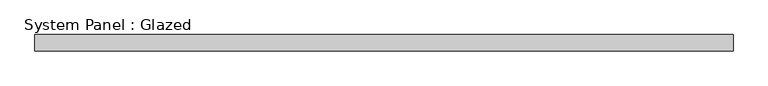
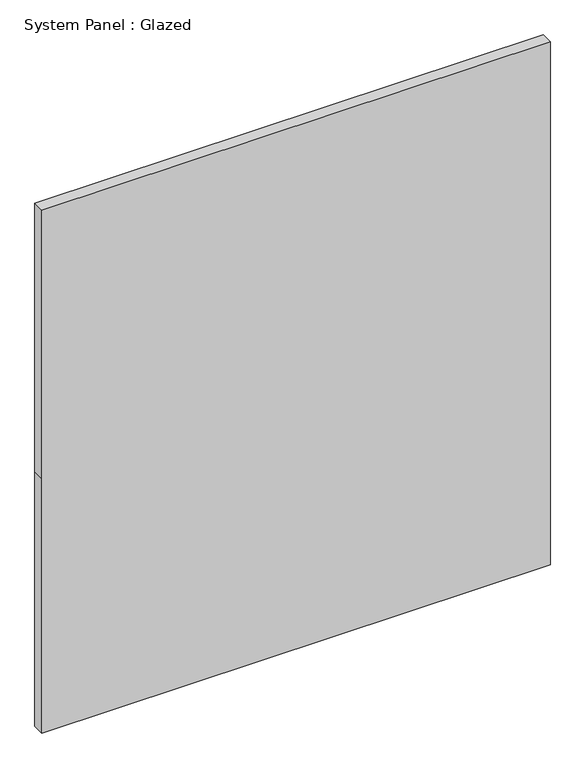
"""IFC4 building model written with IfcOpenShell, lengths in millimetres: plate geometry, System Panel : Glazed."""

import ifcopenshell
import ifcopenshell.guid

model = None  # the IFC model being written
_history = None  # IfcOwnerHistory: only IFC2X3 demands one
_inside = {}  # id of a spatial element -> (the spatial element, [elements in it])
_under = {}  # id of a project, library or spatial element -> (it, [spatial elements below it])
_declared = {}  # id of a project -> (the project, [libraries it declares])
_typed = {}  # id of a type object -> (the type object, [elements of that type])
_made_of = {}  # id of a material, layer set ... -> (it, [elements and type objects made of it])


def new_model(schema):
    """Start an empty IFC model of exactly this schema.

    Asked for "IFC4X3", IfcOpenShell would pick the latest addendum, in which some entities
    have other attributes; the version numbers below select the first issue.
    IFC2X3 requires an IfcOwnerHistory on every rooted entity: one is made here for all.
    """
    global model, _history
    if schema == "IFC4X3":
        model = ifcopenshell.file(schema_version=(4, 3, 0, 0))
    else:
        model = ifcopenshell.file(schema=schema)
    _inside.clear()
    _under.clear()
    _declared.clear()
    _typed.clear()
    _made_of.clear()
    _history = None
    if model.schema == "IFC2X3":
        org = make("IfcOrganization", Name="unknown")
        user = make(
            "IfcPersonAndOrganization",
            ThePerson=make("IfcPerson", FamilyName="unknown"),
            TheOrganization=org,
        )
        app = make(
            "IfcApplication",
            ApplicationDeveloper=org,
            Version="unknown",
            ApplicationFullName="unknown",
            ApplicationIdentifier="unknown",
        )
        _history = make(
            "IfcOwnerHistory",
            OwningUser=user,
            OwningApplication=app,
            ChangeAction="ADDED",
            CreationDate=0,
        )
    return model


def make(cls, **values):
    """One entity of the class cls with the attributes given. An attribute that is None is left unset."""
    return model.create_entity(
        cls, **{name: value for name, value in values.items() if value is not None}
    )


def rooted(cls, **values):
    """An entity with a GlobalId (a new one), such as an element, a storey or a relation."""
    return make(cls, GlobalId=ifcopenshell.guid.new(), OwnerHistory=_history, **values)


def si_unit(unit_type, name, prefix=None):
    """IfcSIUnit, for example si_unit("LENGTHUNIT", "METRE", prefix="MILLI")."""
    return make("IfcSIUnit", UnitType=unit_type, Prefix=prefix, Name=name)


def assignment(units):
    """IfcUnitAssignment: the units of a project."""
    return None if units is None else make("IfcUnitAssignment", Units=units)


def point(xyz):
    """IfcCartesianPoint."""
    return None if xyz is None else make("IfcCartesianPoint", Coordinates=xyz)


def direction(xyz):
    """IfcDirection."""
    return None if xyz is None else make("IfcDirection", DirectionRatios=xyz)


def frame(location, z_axis=None, x_axis=None):
    """IfcAxis2Placement3D, a coordinate frame: its origin and axes. An axis left out is left unset."""
    return make(
        "IfcAxis2Placement3D",
        Location=point(location),
        Axis=direction(z_axis),
        RefDirection=direction(x_axis),
    )


def origin():
    """The frame at (0, 0, 0) with its axes left unset."""
    return frame((0.0, 0.0, 0.0))


def place(relative_to, where):
    """IfcLocalPlacement: puts the frame where relative to a parent placement (None: the world)."""
    return make(
        "IfcLocalPlacement", PlacementRelTo=relative_to, RelativePlacement=where
    )


def context(
    kind, dimensions, precision=None, world=None, true_north=None, identifier=None
):
    """IfcGeometricRepresentationContext, for example the 3D "Model" context."""
    return make(
        "IfcGeometricRepresentationContext",
        ContextIdentifier=identifier,
        ContextType=kind,
        CoordinateSpaceDimension=dimensions,
        Precision=precision,
        WorldCoordinateSystem=world,
        TrueNorth=true_north,
    )


def project(units=None, contexts=None):
    """IfcProject with its units and contexts."""
    return rooted(
        "IfcProject",
        Name="project",
        RepresentationContexts=contexts,
        UnitsInContext=assignment(units),
    )


def spatial(cls, under=None, at=None, **own):
    """A site, building, storey or space (cls), placed at a placement, below another one or the project."""
    s = rooted(cls, ObjectPlacement=at, **own)
    if under is not None:
        _under.setdefault(under.id(), (under, []))[1].append(s)
    return s


def polyline(points):
    """IfcPolyline through the points."""
    return make("IfcPolyline", Points=[point(p) for p in points])


def outline(outer, holes=None, kind="AREA"):
    """IfcArbitraryClosedProfileDef: a profile drawn as a closed curve; with holes, ...WithVoids."""
    if holes is None:
        return make("IfcArbitraryClosedProfileDef", ProfileType=kind, OuterCurve=outer)
    return make(
        "IfcArbitraryProfileDefWithVoids",
        ProfileType=kind,
        OuterCurve=outer,
        InnerCurves=holes,
    )


def extrude(swept, where, along, depth):
    """IfcExtrudedAreaSolid: the profile swept, set in the frame where, extruded along a direction by depth."""
    return make(
        "IfcExtrudedAreaSolid",
        SweptArea=swept,
        Position=where,
        ExtrudedDirection=direction(along),
        Depth=depth,
    )


def shape(context_of_items, identifier, shape_type, items):
    """IfcShapeRepresentation: the items that make up one representation, for example the "Body"."""
    return make(
        "IfcShapeRepresentation",
        ContextOfItems=context_of_items,
        RepresentationIdentifier=identifier,
        RepresentationType=shape_type,
        Items=items,
    )


def source(mapping_origin, context_of_items, identifier, shape_type, items):
    """IfcRepresentationMap: a shape defined once, which mapped items show again and again."""
    return make(
        "IfcRepresentationMap",
        MappingOrigin=mapping_origin,
        MappedRepresentation=shape(context_of_items, identifier, shape_type, items),
    )


def transform(
    local_origin,
    x_axis=None,
    y_axis=None,
    z_axis=None,
    scale=None,
    scale2=None,
    scale3=None,
    uniform=True,
):
    """IfcCartesianTransformationOperator3D, or its non-uniform kind. x_axis, y_axis, z_axis: its Axis1, 2, 3."""
    if uniform:
        return make(
            "IfcCartesianTransformationOperator3D",
            Axis1=direction(x_axis),
            Axis2=direction(y_axis),
            LocalOrigin=point(local_origin),
            Scale=scale,
            Axis3=direction(z_axis),
        )
    return make(
        "IfcCartesianTransformationOperator3DnonUniform",
        Axis1=direction(x_axis),
        Axis2=direction(y_axis),
        LocalOrigin=point(local_origin),
        Scale=scale,
        Axis3=direction(z_axis),
        Scale2=scale2,
        Scale3=scale3,
    )


def mapped(mapping_source, mapping_target):
    """IfcMappedItem: shows the shape of a source again, moved by a transform."""
    return make(
        "IfcMappedItem", MappingSource=mapping_source, MappingTarget=mapping_target
    )


def made_of(thing, what):
    """Note that an element or type object is made of a material, layer set ...; save() writes the relation."""
    if what is not None:
        _made_of.setdefault(what.id(), (what, []))[1].append(thing)
    return thing


def element(
    cls,
    number,
    at=None,
    inside=None,
    cuts=None,
    type_object=None,
    material=None,
    context=None,
    identifier="Body",
    shape_type=None,
    held_by="IfcProductDefinitionShape",
    body=None,
    shapes=None,
    **own,
):
    """One element of the class cls, such as IfcWall. Its Tag is "e" and its number.

    at: its placement. inside: the storey or other place that contains it. cuts: it is an
    opening in that element (IfcRelVoidsElement). A single representation is given by context,
    identifier, shape_type and body (its items); several are given by shapes. held_by: the class
    of the entity that holds the representations. save() writes the other relations.
    """
    e = rooted(cls, Tag="e%d" % number, ObjectPlacement=at, **own)
    if body is not None:
        shapes = [shape(context, identifier, shape_type, body)]
    if shapes is not None:
        e.Representation = make(held_by, Representations=shapes)
    if inside is not None:
        _inside.setdefault(inside.id(), (inside, []))[1].append(e)
    if cuts is not None:
        rooted(
            "IfcRelVoidsElement", RelatingBuildingElement=cuts, RelatedOpeningElement=e
        )
    if type_object is not None:
        _typed.setdefault(type_object.id(), (type_object, []))[1].append(e)
    return made_of(e, material)


def aggregate(whole, parts):
    """IfcRelAggregates: a whole, such as a stair, and the parts it consists of."""
    return rooted("IfcRelAggregates", RelatingObject=whole, RelatedObjects=parts)


def save(model, path):
    """Write the relations noted so far, then the file.

    IfcRelAggregates (storeys below a building ...), IfcRelContainedInSpatialStructure (elements
    in a storey), IfcRelDefinesByType, IfcRelAssociatesMaterial and IfcRelDeclares: one each for
    every whole, place, type object, material and project.
    """
    for whole, parts in _under.values():
        aggregate(whole, parts)
    for where, things in _inside.values():
        rooted(
            "IfcRelContainedInSpatialStructure",
            RelatedElements=things,
            RelatingStructure=where,
        )
    for kind, things in _typed.values():
        rooted("IfcRelDefinesByType", RelatedObjects=things, RelatingType=kind)
    for what, things in _made_of.values():
        rooted("IfcRelAssociatesMaterial", RelatedObjects=things, RelatingMaterial=what)
    for by, libraries in _declared.values():
        rooted("IfcRelDeclares", RelatingContext=by, RelatedDefinitions=libraries)
    model.write(path)


def system_panel_glazed_b3c6389f(model_context):
    return source(origin(), model_context, "Body", "SweptSolid", [
        extrude(outline(polyline([(0.0, -546.4175), (0.0, 546.4175), (577.85, 546.4175), (1187.45, 546.4175), (1187.45, -546.4175), (577.85, -546.4175), (0.0, -546.4175)])), frame((0.0, -44.45, 0.0), z_axis=(0.0, 1.0, 0.0), x_axis=(0.0, 0.0, 1.0)), (0.0, 0.0, 1.0), 25.4),
    ])


if __name__ == "__main__":
    model = new_model("IFC4")
    model_context = context("Model", 3, world=origin())
    ifc_project = project(units=[si_unit("LENGTHUNIT", "METRE", prefix="MILLI")], contexts=[model_context])
    site = spatial("IfcSite", under=ifc_project)
    building = spatial("IfcBuilding", under=site)
    placement = place(None, origin())
    system_panel_glazed_shape = system_panel_glazed_b3c6389f(model_context)
    element("IfcPlate", 1, ObjectType="System Panel : Glazed", at=placement, inside=building, context=model_context, shape_type="MappedRepresentation", body=[
        mapped(system_panel_glazed_shape, transform((0.0, 0.0, 0.0), x_axis=(1.0, 0.0, 0.0), y_axis=(0.0, 1.0, 0.0), z_axis=(0.0, 0.0, 1.0))),
    ])
    save(model, "model.ifc")

# Revit data of these elements
# Element 1 (IfcPlate, "System Panel : Glazed")
#   Materials on its faces: "Glass"
# Materials
#   "Glass": class "Unassigned", colour RGB 0 0 255, transparency 0.75
